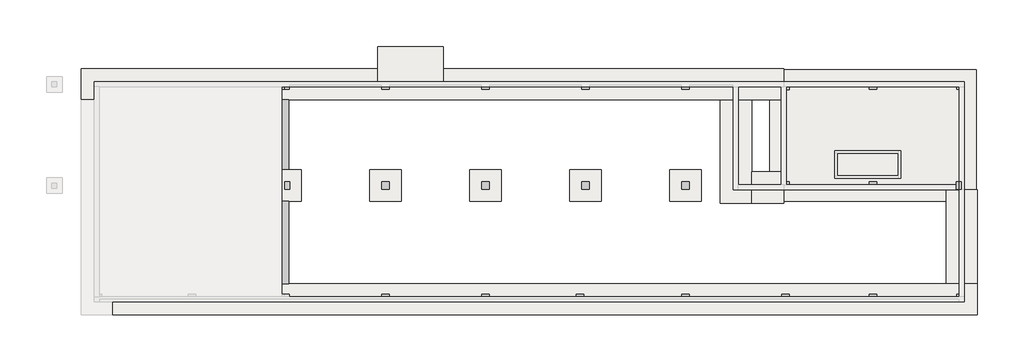
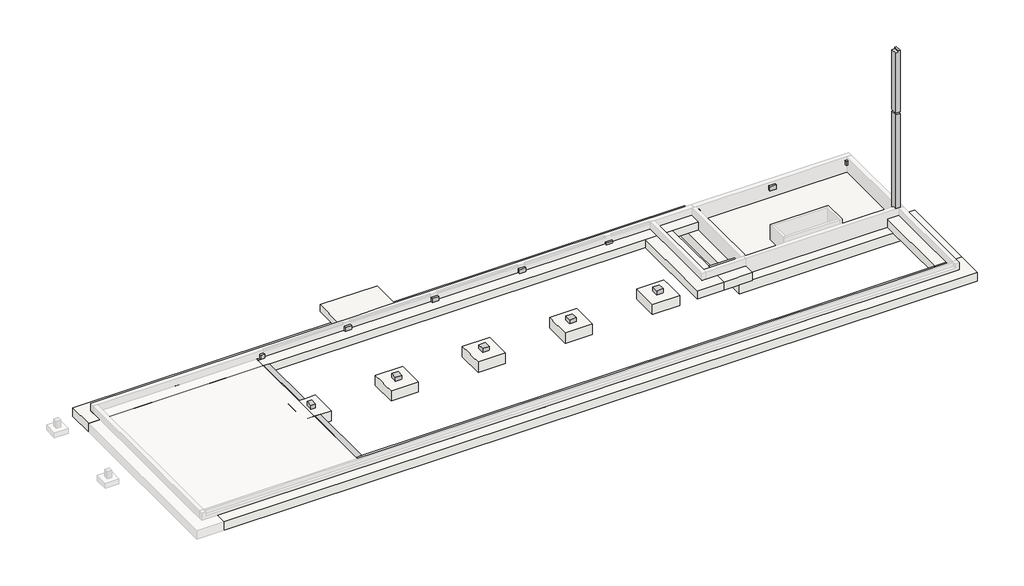
# Not in any storey, part 2 of 2: 25 columns, 8 beams, 8 slabs, 5 footings.
# Revit data of these elements (continued)
# Type "H_SF_AR_B01_MAT_Bitumen_MF2" (continued)
#   H_WM Code_3 = "A03AF036-00001 |  | M2 | Concrete Work | Superstructure Work | Form Work (1 time in use) | Flat Form | Dressed Lumber, Plywood or Steel Form(Wood Planks are not Allowed) incl. Chamfer |  |  |  | A03AF036-00001 Concrete Work Superstructure Work Form Work (1 time in use) Flat Form     Dressed Lumber, Plywood or Steel Form(Wood Planks are not Allowed) incl. Chamfer   |"
#   H_Rebar ratio = 0.12
#   Layers, outside or top first: 650 mm "00_Concrete_Reinf. Conc." (function 1)
# Type "Foundation Rectangular (Non-Pile) : H_SF_AR_S18_W2500xL2500xT1000_Bitumen_F1"
#   Type Comments = "CV-UG"
#   Type Mark = "F1"
#   H_Q'ty Cal Type Tag = "SC-Q1A"
#   H_WM Code_1 = "A03AD044-00001 |  | M | Concrete Work | Substructure Work | Isolation Joint (Separation Joint) | w/ Flexible Joint Filler, Sealant | THK=(  )mm |  | A03AD044-00001 Concrete Work Substructure Work Isolation Joint (Separation Joint)      w/ Flexible Joint Filler, Sealant   | THK=( 12 )mm"
#   H_WM Code_2 = "A03AD032-00022 |  | M3 | Concrete Work | Substructure Work | Structural Concrete | Cement Type-1 | 25MPa ≤ F'c (Cylinder Strength) < 30MPa |  |  |  |  | A03AD032-00022 Concrete Work Substructure Work Structural Concrete  Cement Type-1 25MPa ≤ F'c (Cylinder Strength) < 30MPa      |  F'c (Cylinder Strength) = 24MPa"
#   H_WM Code_3 = "A03AD037-00002 |  | TON | Concrete Work | Substructure Work | Rebar Work | Deformed Bar (Non-Coat.) | 400MPa<Fy≤470MPa |  |  |  |  | A03AD037-00002 Concrete Work Substructure Work Rebar Work Deformed Bar (Non-Coat.)  400MPa<Fy≤470MPa      | ASTM A615 GRADE 60 (Fy=420MPa)"
#   H_WM Code_4 = "A03AD035-00001 |  | M2 | Concrete Work | Substructure Work | Form Work (3 times in use) | Flat Form | Dressed Lumber, Plywood or Steel Form(Wood Planks are not Allowed) incl. Chamfer |  |  |  | A03AD035-00001 Concrete Work Substructure Work Form Work (3 times in use) Flat Form     Dressed Lumber, Plywood or Steel Form(Wood Planks are not Allowed) incl. Chamfer   |"
#   H_WM Code_5 = "A01ZZ003-00001 |  | M3 | Earth Work | - | Backfill | Re-use, Soil |  |  |  | Compaction=(  )% |  | A01ZZ003-00001 Earth Work - Backfill Re-use, Soil        | Compaction=( 95 )%"
#   H_WM Code_6 = "A01ZZ004-00001 |  | M3 | Earth Work | - | Disposal | Soil |  |  |  | Disposal Distance=Appx. (  )km from Site |  | A01ZZ004-00001 Earth Work - Disposal Soil        | Disposal Distance=Appx. (20 )km from Site"
#   H_WM Code_7 = "A03AH056-00001 |  | M2 | Concrete Work | Concrete Protective Coating (U/G) | Bitumen/Bituminous/Asphalt Coating |  |  | A03AH056-00001 Concrete Work Concrete Protective Coating (U/G) Bitumen/Bituminous/Asphalt Coating         |"
#   Top bar = "D25@300"
#   Description = "UG Shallow Foundation"
#   Bottom bar = "D20@300"
#   H_Rebar ratio = 0.12
#   Width = 2500 mm
#   Length = 2500 mm
#   Foundation Thickness = 1000 mm
#   Structural Material [instance default] = none
#   Assembly Code = ""
# Elements 1, 2 (IfcBeam, "RC Beam_Rectangular : H_SB_AR_S16_TG_B600xH800_FG2")
#   Comments = ""
#   hec_material3 = none
#   hec_material2 = none
#   hec_material1 = 00_Concrete_Reinf. Conc.
#   Structural Material = 00_Concrete_Reinf. Conc.
#   Phase Created = New Construction
#   Materials on its faces: "00_Concrete_Reinf. Conc."
# Elements 3, 4, 5 (IfcBeam, "RC Beam_Rectangular : H_SB_AR_S16_TG_B500xH700_FB1")
#   Comments = ""
#   hec_material3 = none
#   hec_material2 = none
#   hec_material1 = none
#   Structural Material = 00_Concrete_Reinf. Conc.
#   Phase Created = New Construction
#   Materials on its faces: "00_Concrete_Reinf. Conc."
# Elements 6, 7, 8 (IfcBeam, "RC Beam_Rectangular : H_SB_AR_S16_TG_B500xH700_FG1")
#   Comments = ""
#   hec_material3 = none
#   hec_material2 = none
#   hec_material1 = none
#   Structural Material = 00_Concrete_Reinf. Conc.
#   Phase Created = New Construction
#   Materials on its faces: "00_Concrete_Reinf. Conc."
# Element 9 (IfcColumn, "RC_Column_Rectangular : H_SC_AR_S15_UG_W600xL600_C2")
#   Comments = ""
#   H_Re Bar Ratio = 0.3
#   hec_material3 = none
#   hec_material2 = none
#   hec_material1 = none
#   Structural Material = 00_Concrete_Reinf. Conc.
#   Phase Created = New Construction
#   Materials on its faces: "00_Concrete_Reinf. Conc."
# Elements 10, 11, 12, 13, 14, 15, 16, 17, 18, 19, 20, 21, 22, 31, 32 (IfcColumn, "RC_Column_Rectangular : H_SC_AR_S15_UG_W600xL600_C2")
#   Comments = ""
#   hec_material3 = none
#   hec_material2 = none
#   hec_material1 = none
#   Structural Material = 00_Concrete_Reinf. Conc.
#   Phase Created = New Construction
#   Materials on its faces: "00_Concrete_Reinf. Conc."
# Elements 23, 24, 25, 26, 27, 28, 29, 30, 33 (IfcColumn, "RC_Column_Rectangular : H_SC_AR_S15_AG_W600xL600_C2")
#   Comments = ""
#   hec_material3 = none
#   hec_material2 = none
#   hec_material1 = none
#   Structural Material = 00_Concrete_Reinf. Conc.
#   Phase Created = New Construction
#   Materials on its faces: "00_Concrete_Reinf. Conc."
# Elements 34, 37, 38 (IfcFooting, "H_SF_AR_S18_Wall FDN_T800")
#   Comments = ""
#   Phase Created = New Construction
#   Materials on its faces: "00_Concrete_Reinf. Conc."
# Element 35 (IfcFooting, "H_SF_AR_S18_Wall FDN_T800")
#   Comments = ""
#   H_Re Bar Ratio = 0.3
#   Phase Created = New Construction
#   Materials on its faces: "00_Concrete_Reinf. Conc."
# Element 36 (IfcFooting, "H_SF_AR_S18_Wall FDN_T800")
#   Phase Created = New Construction
#   Materials on its faces: "00_Concrete_Reinf. Conc."
# Element 39 (IfcSlab, "H_SF_AR_B01_MAT_Bitumen_MF1")
#   Comments = ""
#   Height Offset From Level = 0 mm
#   built-in parameter 1001954 = 1
#   Phase Created = New Construction
#   Materials on its faces: "00_Concrete_Reinf. Conc."
# Element 40 (IfcSlab, "H_SF_AR_B01_MAT_Bitumen_MF2")
#   Comments = ""
#   Height Offset From Level = 1450 mm
#   built-in parameter 1001954 = 1
#   Phase Created = New Construction
#   Materials on its faces: "00_Concrete_Reinf. Conc."
# Elements 41, 42, 43, 44, 45, 46 (IfcSlab, "Foundation Rectangular (Non-Pile) : H_SF_AR_S18_W2500xL2500xT1000_Bitumen_F1")
#   Comments = ""
#   Structural Material = 00_Concrete_Reinf. Conc.
#   Phase Created = New Construction
#   Materials on its faces: "00_Concrete_Reinf. Conc."
# Materials
#   "00_Concrete_Reinf. Conc.": class "Concrete", colour RGB 176 176 176, transparency 0, Description = "Reinf. Conc.", Cost = 0, Image = Concrete.Cast-In-Place.Flat.Polished.Grey.jpg
